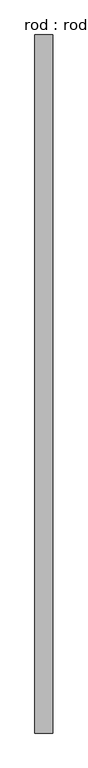
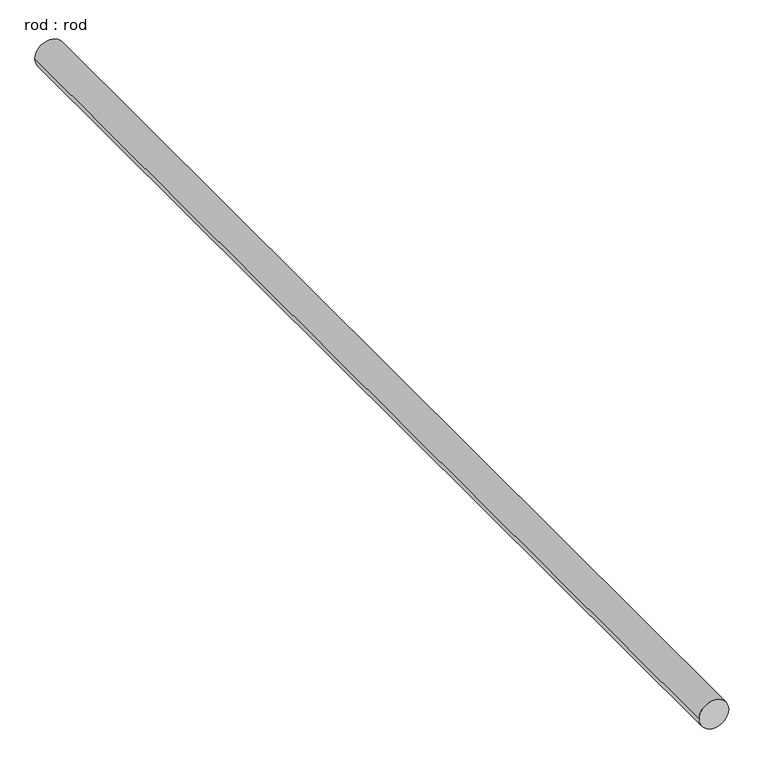
"""IFC4 building model written with IfcOpenShell, lengths in millimetres: proxy geometry, rod : rod."""

from ifc_helpers import new_model, si_unit, point, frame, frame_2d, origin, place, context, project, spatial, circle_curve, trimmed, segment, composite_curve, outline, extrude, source, transform, mapped, element, save


def rod_rod_212dde4f(model_context):
    return source(origin(), model_context, "Body", "SweptSolid", [
        extrude(outline(composite_curve([segment(trimmed(circle_curve(frame_2d((0.0108462, 0.0)), 200.0), [point((0.0108462, 200.0))], [point((0.0108462, -200.0))], False, "CARTESIAN"), True, "CONTINUOUS"), segment(trimmed(circle_curve(frame_2d((0.0108462, 0.0)), 200.0), [point((0.0108462, -200.0))], [point((0.0108462, 200.0))], False, "CARTESIAN"), True, "CONTINUOUS")], self_intersect=False)), frame((0.0, -3684.3185577, 0.0), z_axis=(0.0, 1.0, 0.0), x_axis=(0.0, 0.0, 1.0)), (0.0, 0.0, 1.0), 15554.094346),
    ])


if __name__ == "__main__":
    model = new_model("IFC4")
    model_context = context("Model", 3, world=origin())
    ifc_project = project(units=[si_unit("LENGTHUNIT", "METRE", prefix="MILLI")], contexts=[model_context])
    site = spatial("IfcSite", under=ifc_project)
    building = spatial("IfcBuilding", under=site)
    placement = place(None, origin())
    rod_rod_shape = rod_rod_212dde4f(model_context)
    element("IfcBuildingElementProxy", 1, Name="rod : rod", ObjectType="rod : rod", at=placement, inside=building, context=model_context, shape_type="MappedRepresentation", body=[
        mapped(rod_rod_shape, transform((0.0, 0.0, 0.0), x_axis=(1.0, 0.0, 0.0), y_axis=(0.0, 1.0, 0.0), z_axis=(0.0, 0.0, 1.0))),
    ])
    save(model, "model.ifc")

# Revit data of these elements
# Type "rod : rod"
#   Default Elevation = 0
